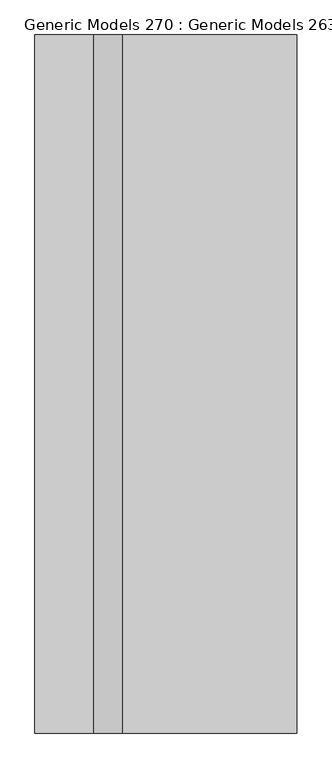
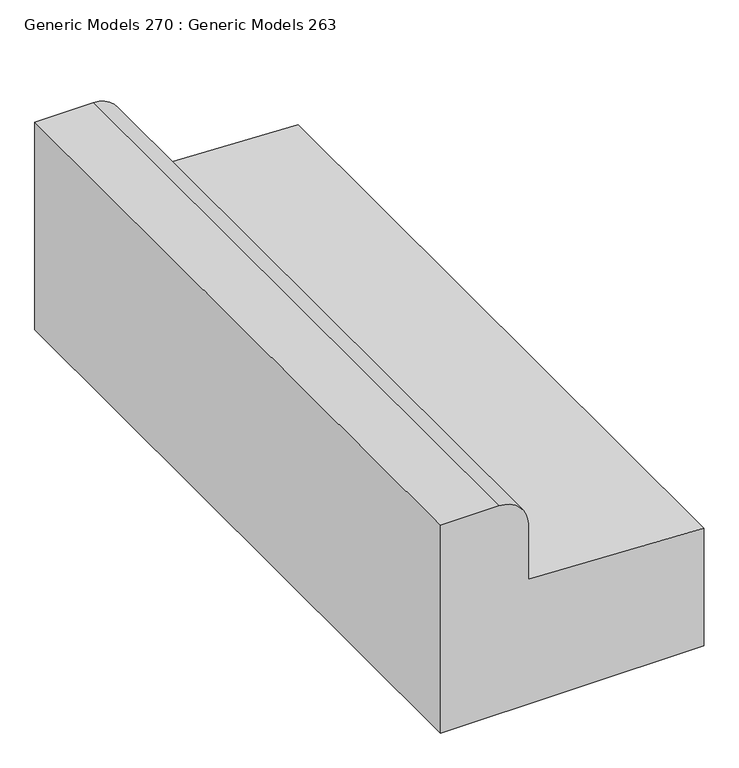
"""IFC4 building model written with IfcOpenShell, lengths in millimetres: proxy geometry, Generic Models 270 : Generic Models 263."""

import ifcopenshell
import ifcopenshell.guid

model = None  # the IFC model being written
_history = None  # IfcOwnerHistory: only IFC2X3 demands one
_inside = {}  # id of a spatial element -> (the spatial element, [elements in it])
_under = {}  # id of a project, library or spatial element -> (it, [spatial elements below it])
_declared = {}  # id of a project -> (the project, [libraries it declares])
_typed = {}  # id of a type object -> (the type object, [elements of that type])
_made_of = {}  # id of a material, layer set ... -> (it, [elements and type objects made of it])


def new_model(schema):
    """Start an empty IFC model of exactly this schema.

    Asked for "IFC4X3", IfcOpenShell would pick the latest addendum, in which some entities
    have other attributes; the version numbers below select the first issue.
    IFC2X3 requires an IfcOwnerHistory on every rooted entity: one is made here for all.
    """
    global model, _history
    if schema == "IFC4X3":
        model = ifcopenshell.file(schema_version=(4, 3, 0, 0))
    else:
        model = ifcopenshell.file(schema=schema)
    _inside.clear()
    _under.clear()
    _declared.clear()
    _typed.clear()
    _made_of.clear()
    _history = None
    if model.schema == "IFC2X3":
        org = make("IfcOrganization", Name="unknown")
        user = make(
            "IfcPersonAndOrganization",
            ThePerson=make("IfcPerson", FamilyName="unknown"),
            TheOrganization=org,
        )
        app = make(
            "IfcApplication",
            ApplicationDeveloper=org,
            Version="unknown",
            ApplicationFullName="unknown",
            ApplicationIdentifier="unknown",
        )
        _history = make(
            "IfcOwnerHistory",
            OwningUser=user,
            OwningApplication=app,
            ChangeAction="ADDED",
            CreationDate=0,
        )
    return model


def make(cls, **values):
    """One entity of the class cls with the attributes given. An attribute that is None is left unset."""
    return model.create_entity(
        cls, **{name: value for name, value in values.items() if value is not None}
    )


def rooted(cls, **values):
    """An entity with a GlobalId (a new one), such as an element, a storey or a relation."""
    return make(cls, GlobalId=ifcopenshell.guid.new(), OwnerHistory=_history, **values)


def si_unit(unit_type, name, prefix=None):
    """IfcSIUnit, for example si_unit("LENGTHUNIT", "METRE", prefix="MILLI")."""
    return make("IfcSIUnit", UnitType=unit_type, Prefix=prefix, Name=name)


def assignment(units):
    """IfcUnitAssignment: the units of a project."""
    return None if units is None else make("IfcUnitAssignment", Units=units)


def point(xyz):
    """IfcCartesianPoint."""
    return None if xyz is None else make("IfcCartesianPoint", Coordinates=xyz)


def direction(xyz):
    """IfcDirection."""
    return None if xyz is None else make("IfcDirection", DirectionRatios=xyz)


def frame(location, z_axis=None, x_axis=None):
    """IfcAxis2Placement3D, a coordinate frame: its origin and axes. An axis left out is left unset."""
    return make(
        "IfcAxis2Placement3D",
        Location=point(location),
        Axis=direction(z_axis),
        RefDirection=direction(x_axis),
    )


def frame_2d(location, x_axis=None):
    """IfcAxis2Placement2D, a coordinate frame in the plane: its origin and x axis."""
    return make(
        "IfcAxis2Placement2D", Location=point(location), RefDirection=direction(x_axis)
    )


def origin():
    """The frame at (0, 0, 0) with its axes left unset."""
    return frame((0.0, 0.0, 0.0))


def place(relative_to, where):
    """IfcLocalPlacement: puts the frame where relative to a parent placement (None: the world)."""
    return make(
        "IfcLocalPlacement", PlacementRelTo=relative_to, RelativePlacement=where
    )


def context(
    kind, dimensions, precision=None, world=None, true_north=None, identifier=None
):
    """IfcGeometricRepresentationContext, for example the 3D "Model" context."""
    return make(
        "IfcGeometricRepresentationContext",
        ContextIdentifier=identifier,
        ContextType=kind,
        CoordinateSpaceDimension=dimensions,
        Precision=precision,
        WorldCoordinateSystem=world,
        TrueNorth=true_north,
    )


def project(units=None, contexts=None):
    """IfcProject with its units and contexts."""
    return rooted(
        "IfcProject",
        Name="project",
        RepresentationContexts=contexts,
        UnitsInContext=assignment(units),
    )


def spatial(cls, under=None, at=None, **own):
    """A site, building, storey or space (cls), placed at a placement, below another one or the project."""
    s = rooted(cls, ObjectPlacement=at, **own)
    if under is not None:
        _under.setdefault(under.id(), (under, []))[1].append(s)
    return s


def polyline(points):
    """IfcPolyline through the points."""
    return make("IfcPolyline", Points=[point(p) for p in points])


def circle_curve(where, radius):
    """IfcCircle in the frame where."""
    return make("IfcCircle", Position=where, Radius=radius)


def trimmed(basis, trim1, trim2, sense, master):
    """IfcTrimmedCurve: the piece of a basis curve between two trims."""
    return make(
        "IfcTrimmedCurve",
        BasisCurve=basis,
        Trim1=trim1,
        Trim2=trim2,
        SenseAgreement=sense,
        MasterRepresentation=master,
    )


def segment(curve, same_sense, transition):
    """IfcCompositeCurveSegment."""
    return make(
        "IfcCompositeCurveSegment",
        Transition=transition,
        SameSense=same_sense,
        ParentCurve=curve,
    )


def composite_curve(segments, self_intersect=None):
    """IfcCompositeCurve: segments joined end to end."""
    return make("IfcCompositeCurve", Segments=segments, SelfIntersect=self_intersect)


def outline(outer, holes=None, kind="AREA"):
    """IfcArbitraryClosedProfileDef: a profile drawn as a closed curve; with holes, ...WithVoids."""
    if holes is None:
        return make("IfcArbitraryClosedProfileDef", ProfileType=kind, OuterCurve=outer)
    return make(
        "IfcArbitraryProfileDefWithVoids",
        ProfileType=kind,
        OuterCurve=outer,
        InnerCurves=holes,
    )


def extrude(swept, where, along, depth):
    """IfcExtrudedAreaSolid: the profile swept, set in the frame where, extruded along a direction by depth."""
    return make(
        "IfcExtrudedAreaSolid",
        SweptArea=swept,
        Position=where,
        ExtrudedDirection=direction(along),
        Depth=depth,
    )


def shape(context_of_items, identifier, shape_type, items):
    """IfcShapeRepresentation: the items that make up one representation, for example the "Body"."""
    return make(
        "IfcShapeRepresentation",
        ContextOfItems=context_of_items,
        RepresentationIdentifier=identifier,
        RepresentationType=shape_type,
        Items=items,
    )


def source(mapping_origin, context_of_items, identifier, shape_type, items):
    """IfcRepresentationMap: a shape defined once, which mapped items show again and again."""
    return make(
        "IfcRepresentationMap",
        MappingOrigin=mapping_origin,
        MappedRepresentation=shape(context_of_items, identifier, shape_type, items),
    )


def transform(
    local_origin,
    x_axis=None,
    y_axis=None,
    z_axis=None,
    scale=None,
    scale2=None,
    scale3=None,
    uniform=True,
):
    """IfcCartesianTransformationOperator3D, or its non-uniform kind. x_axis, y_axis, z_axis: its Axis1, 2, 3."""
    if uniform:
        return make(
            "IfcCartesianTransformationOperator3D",
            Axis1=direction(x_axis),
            Axis2=direction(y_axis),
            LocalOrigin=point(local_origin),
            Scale=scale,
            Axis3=direction(z_axis),
        )
    return make(
        "IfcCartesianTransformationOperator3DnonUniform",
        Axis1=direction(x_axis),
        Axis2=direction(y_axis),
        LocalOrigin=point(local_origin),
        Scale=scale,
        Axis3=direction(z_axis),
        Scale2=scale2,
        Scale3=scale3,
    )


def mapped(mapping_source, mapping_target):
    """IfcMappedItem: shows the shape of a source again, moved by a transform."""
    return make(
        "IfcMappedItem", MappingSource=mapping_source, MappingTarget=mapping_target
    )


def made_of(thing, what):
    """Note that an element or type object is made of a material, layer set ...; save() writes the relation."""
    if what is not None:
        _made_of.setdefault(what.id(), (what, []))[1].append(thing)
    return thing


def element(
    cls,
    number,
    at=None,
    inside=None,
    cuts=None,
    type_object=None,
    material=None,
    context=None,
    identifier="Body",
    shape_type=None,
    held_by="IfcProductDefinitionShape",
    body=None,
    shapes=None,
    **own,
):
    """One element of the class cls, such as IfcWall. Its Tag is "e" and its number.

    at: its placement. inside: the storey or other place that contains it. cuts: it is an
    opening in that element (IfcRelVoidsElement). A single representation is given by context,
    identifier, shape_type and body (its items); several are given by shapes. held_by: the class
    of the entity that holds the representations. save() writes the other relations.
    """
    e = rooted(cls, Tag="e%d" % number, ObjectPlacement=at, **own)
    if body is not None:
        shapes = [shape(context, identifier, shape_type, body)]
    if shapes is not None:
        e.Representation = make(held_by, Representations=shapes)
    if inside is not None:
        _inside.setdefault(inside.id(), (inside, []))[1].append(e)
    if cuts is not None:
        rooted(
            "IfcRelVoidsElement", RelatingBuildingElement=cuts, RelatedOpeningElement=e
        )
    if type_object is not None:
        _typed.setdefault(type_object.id(), (type_object, []))[1].append(e)
    return made_of(e, material)


def aggregate(whole, parts):
    """IfcRelAggregates: a whole, such as a stair, and the parts it consists of."""
    return rooted("IfcRelAggregates", RelatingObject=whole, RelatedObjects=parts)


def save(model, path):
    """Write the relations noted so far, then the file.

    IfcRelAggregates (storeys below a building ...), IfcRelContainedInSpatialStructure (elements
    in a storey), IfcRelDefinesByType, IfcRelAssociatesMaterial and IfcRelDeclares: one each for
    every whole, place, type object, material and project.
    """
    for whole, parts in _under.values():
        aggregate(whole, parts)
    for where, things in _inside.values():
        rooted(
            "IfcRelContainedInSpatialStructure",
            RelatedElements=things,
            RelatingStructure=where,
        )
    for kind, things in _typed.values():
        rooted("IfcRelDefinesByType", RelatedObjects=things, RelatingType=kind)
    for what, things in _made_of.values():
        rooted("IfcRelAssociatesMaterial", RelatedObjects=things, RelatingMaterial=what)
    for by, libraries in _declared.values():
        rooted("IfcRelDeclares", RelatingContext=by, RelatedDefinitions=libraries)
    model.write(path)


def generic_models_270_generic_models_263_c5a2dacb(model_context):
    return source(origin(), model_context, "Body", "SweptSolid", [
        extrude(outline(composite_curve([segment(polyline([(0.0, 62420.7797726), (0.0, 62319.1797726), (-381.0, 62319.1797726), (-381.0, 62776.3797726), (-165.1, 62776.3797726), (-152.4, 62471.5797726), (-50.8, 62471.5797726)]), True, "CONTINUOUS"), segment(trimmed(circle_curve(frame_2d((-50.8, 62420.7797726)), 50.8), [point((-50.8, 62471.5797726))], [point((0.0, 62420.7797726))], False, "CARTESIAN"), True, "CONTINUOUS")], self_intersect=False)), frame((0.0, -94.4486541, 0.0), z_axis=(0.0, 1.0, 0.0), x_axis=(0.0, 0.0, 1.0)), (0.0, 0.0, 1.0), 1219.2),
    ])


if __name__ == "__main__":
    model = new_model("IFC4")
    model_context = context("Model", 3, world=origin())
    ifc_project = project(units=[si_unit("LENGTHUNIT", "METRE", prefix="MILLI")], contexts=[model_context])
    site = spatial("IfcSite", under=ifc_project)
    building = spatial("IfcBuilding", under=site)
    placement = place(None, origin())
    generic_models_270_generic_models_263_shape = generic_models_270_generic_models_263_c5a2dacb(model_context)
    element("IfcBuildingElementProxy", 1, Name="Generic Models 270 : Generic Models 263", ObjectType="Generic Models 270 : Generic Models 263", at=placement, inside=building, context=model_context, shape_type="MappedRepresentation", body=[
        mapped(generic_models_270_generic_models_263_shape, transform((0.0, 0.0, 0.0), x_axis=(1.0, 0.0, 0.0), y_axis=(0.0, 1.0, 0.0), z_axis=(0.0, 0.0, 1.0))),
    ])
    save(model, "model.ifc")

# Revit data of these elements
# Element 1 (IfcBuildingElementProxy, "Generic Models 270 : Generic Models 263")
#   Materials on its faces: "CONCRETE CURB"
# Materials
#   "CONCRETE CURB": class "Concrete", colour RGB 191 191 191, transparency 0, Description = "Cast-in-place concrete", Cost = 0
